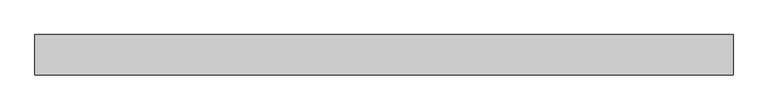
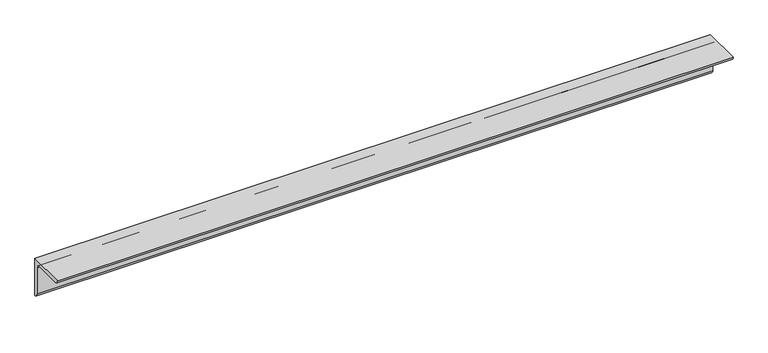
"""IFC4 building model written with IfcOpenShell, lengths in millimetres: member geometry, 0912_Steel Framing_L-KSD3502 : H_SB_AR_S04_L-100x100x10_KBR2."""

from ifc_helpers import new_model, si_unit, point, frame, frame_2d, origin, place, context, project, spatial, polyline, circle_curve, trimmed, segment, composite_curve, outline, extrude, source, transform, mapped, element, save


def member_7f428fab(model_context):
    return source(origin(), model_context, "Body", "SweptSolid", [
        extrude(outline(composite_curve([segment(polyline([(28.2, 28.2), (28.2, -71.8)]), True, "CONTINUOUS"), segment(trimmed(circle_curve(frame_2d((28.2, -61.8)), 10.0), [point((28.2, -71.8))], [point((18.2, -61.8))], False, "CARTESIAN"), True, "CONTINUOUS"), segment(polyline([(18.2, -61.8), (18.2, 8.2)]), True, "CONTINUOUS"), segment(trimmed(circle_curve(frame_2d((8.2, 8.2)), 10.0), [point((18.2, 8.2))], [point((8.2, 18.2))], True, "CARTESIAN"), True, "CONTINUOUS"), segment(polyline([(8.2, 18.2), (-61.8, 18.2)]), True, "CONTINUOUS"), segment(trimmed(circle_curve(frame_2d((-61.8, 28.2)), 10.0), [point((-61.8, 18.2))], [point((-71.8, 28.2))], False, "CARTESIAN"), True, "CONTINUOUS"), segment(polyline([(-71.8, 28.2), (28.2, 28.2)]), True, "CONTINUOUS")], self_intersect=False)), frame((-853.0825032, 0.0, 0.0), z_axis=(1.0, 0.0, 0.0), x_axis=(0.0, 1.0, 0.0)), (0.0, 0.0, 1.0), 1723.8034376),
    ])


if __name__ == "__main__":
    model = new_model("IFC4")
    model_context = context("Model", 3, world=origin())
    ifc_project = project(units=[si_unit("LENGTHUNIT", "METRE", prefix="MILLI")], contexts=[model_context])
    site = spatial("IfcSite", under=ifc_project)
    building = spatial("IfcBuilding", under=site)
    placement = place(None, origin())
    member_shape = member_7f428fab(model_context)
    element("IfcMember", 1, ObjectType="0912_Steel Framing_L-KSD3502 : H_SB_AR_S04_L-100x100x10_KBR2", at=placement, inside=building, context=model_context, shape_type="MappedRepresentation", body=[
        mapped(member_shape, transform((0.0, 0.0, 0.0), x_axis=(1.0, 0.0, 0.0), y_axis=(0.0, 1.0, 0.0), z_axis=(0.0, 0.0, 1.0))),
    ])
    save(model, "model.ifc")

# Revit data of these elements
# Type "0912_Steel Framing_L-KSD3502 : H_SB_AR_S04_L-100x100x10_KBR2"
#   k = 25 mm
#   Perimeter = 0.40 m²/m
#   Nominal Weight = 14.90 kgf/m
#   Length [instance default] = 1000 mm
#   b = 100 mm
#   d = 100 mm
#   t = 10 mm
#   x = 28.2 mm
#   y = 28.2 mm
#   A = 1900.00 m²
#   Structural Material [instance default] = Steel, 45-345
# Element 1 (IfcMember, "0912_Steel Framing_L-KSD3502 : H_SB_AR_S04_L-100x100x10_KBR2")
#   Materials on its faces: "Steel, 45-345"
# Materials
#   "Steel, 45-345": class "Metal", colour RGB 189 187 185, transparency 0, Description = "Steel 345 MPa", Cost = 0
